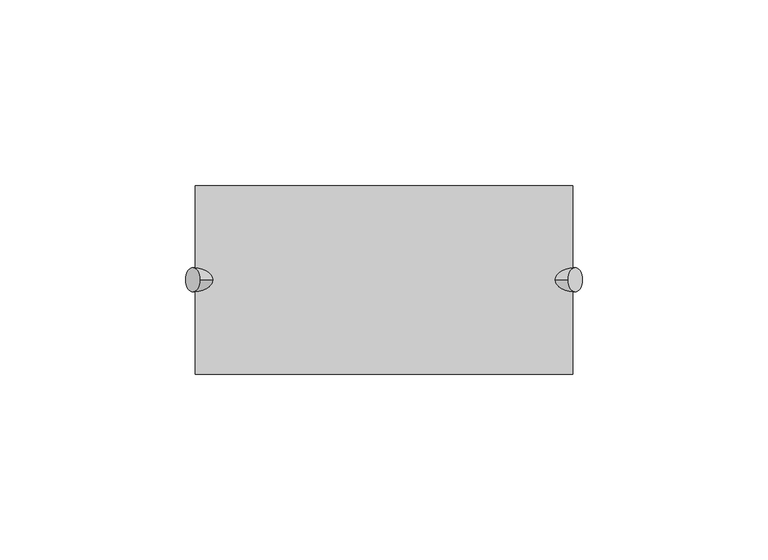
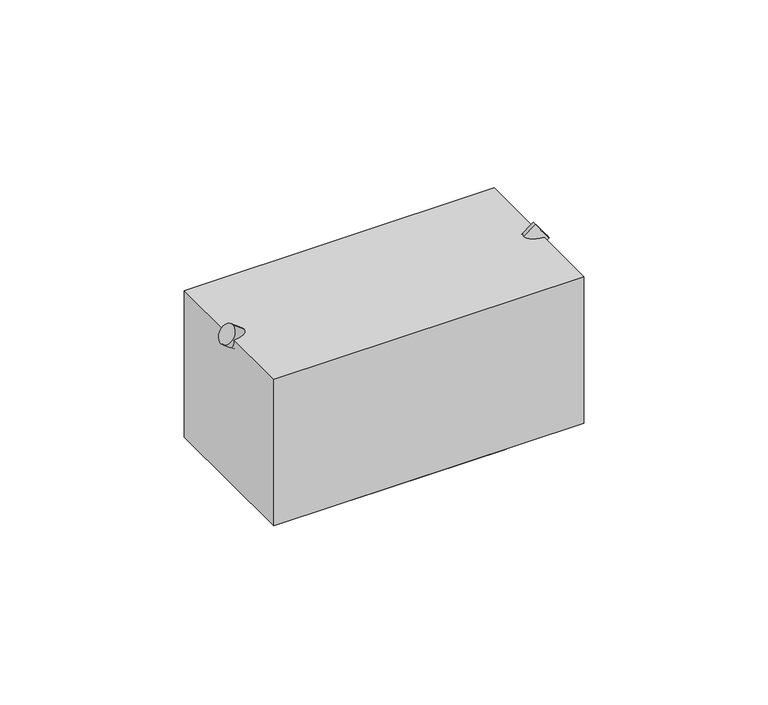
"""IFC4 building model written with IfcOpenShell, lengths in millimetres: proxy geometry, A5145 - Hook, Garment, Double : A5145 - Hook, Garment, Double."""

import ifcopenshell
import ifcopenshell.guid

model = None  # the IFC model being written
_history = None  # IfcOwnerHistory: only IFC2X3 demands one
_inside = {}  # id of a spatial element -> (the spatial element, [elements in it])
_under = {}  # id of a project, library or spatial element -> (it, [spatial elements below it])
_declared = {}  # id of a project -> (the project, [libraries it declares])
_typed = {}  # id of a type object -> (the type object, [elements of that type])
_made_of = {}  # id of a material, layer set ... -> (it, [elements and type objects made of it])


def new_model(schema):
    """Start an empty IFC model of exactly this schema.

    Asked for "IFC4X3", IfcOpenShell would pick the latest addendum, in which some entities
    have other attributes; the version numbers below select the first issue.
    IFC2X3 requires an IfcOwnerHistory on every rooted entity: one is made here for all.
    """
    global model, _history
    if schema == "IFC4X3":
        model = ifcopenshell.file(schema_version=(4, 3, 0, 0))
    else:
        model = ifcopenshell.file(schema=schema)
    _inside.clear()
    _under.clear()
    _declared.clear()
    _typed.clear()
    _made_of.clear()
    _history = None
    if model.schema == "IFC2X3":
        org = make("IfcOrganization", Name="unknown")
        user = make(
            "IfcPersonAndOrganization",
            ThePerson=make("IfcPerson", FamilyName="unknown"),
            TheOrganization=org,
        )
        app = make(
            "IfcApplication",
            ApplicationDeveloper=org,
            Version="unknown",
            ApplicationFullName="unknown",
            ApplicationIdentifier="unknown",
        )
        _history = make(
            "IfcOwnerHistory",
            OwningUser=user,
            OwningApplication=app,
            ChangeAction="ADDED",
            CreationDate=0,
        )
    return model


def make(cls, **values):
    """One entity of the class cls with the attributes given. An attribute that is None is left unset."""
    return model.create_entity(
        cls, **{name: value for name, value in values.items() if value is not None}
    )


def rooted(cls, **values):
    """An entity with a GlobalId (a new one), such as an element, a storey or a relation."""
    return make(cls, GlobalId=ifcopenshell.guid.new(), OwnerHistory=_history, **values)


def si_unit(unit_type, name, prefix=None):
    """IfcSIUnit, for example si_unit("LENGTHUNIT", "METRE", prefix="MILLI")."""
    return make("IfcSIUnit", UnitType=unit_type, Prefix=prefix, Name=name)


def assignment(units):
    """IfcUnitAssignment: the units of a project."""
    return None if units is None else make("IfcUnitAssignment", Units=units)


def point(xyz):
    """IfcCartesianPoint."""
    return None if xyz is None else make("IfcCartesianPoint", Coordinates=xyz)


def direction(xyz):
    """IfcDirection."""
    return None if xyz is None else make("IfcDirection", DirectionRatios=xyz)


def frame(location, z_axis=None, x_axis=None):
    """IfcAxis2Placement3D, a coordinate frame: its origin and axes. An axis left out is left unset."""
    return make(
        "IfcAxis2Placement3D",
        Location=point(location),
        Axis=direction(z_axis),
        RefDirection=direction(x_axis),
    )


def origin():
    """The frame at (0, 0, 0) with its axes left unset."""
    return frame((0.0, 0.0, 0.0))


def origin_with_axes():
    """The frame at (0, 0, 0) with the z axis (0, 0, 1) and the x axis (1, 0, 0) written out."""
    return frame((0.0, 0.0, 0.0), z_axis=(0.0, 0.0, 1.0), x_axis=(1.0, 0.0, 0.0))


def place(relative_to, where):
    """IfcLocalPlacement: puts the frame where relative to a parent placement (None: the world)."""
    return make(
        "IfcLocalPlacement", PlacementRelTo=relative_to, RelativePlacement=where
    )


def context(
    kind, dimensions, precision=None, world=None, true_north=None, identifier=None
):
    """IfcGeometricRepresentationContext, for example the 3D "Model" context."""
    return make(
        "IfcGeometricRepresentationContext",
        ContextIdentifier=identifier,
        ContextType=kind,
        CoordinateSpaceDimension=dimensions,
        Precision=precision,
        WorldCoordinateSystem=world,
        TrueNorth=true_north,
    )


def project(units=None, contexts=None):
    """IfcProject with its units and contexts."""
    return rooted(
        "IfcProject",
        Name="project",
        RepresentationContexts=contexts,
        UnitsInContext=assignment(units),
    )


def spatial(cls, under=None, at=None, **own):
    """A site, building, storey or space (cls), placed at a placement, below another one or the project."""
    s = rooted(cls, ObjectPlacement=at, **own)
    if under is not None:
        _under.setdefault(under.id(), (under, []))[1].append(s)
    return s


def polyline(points):
    """IfcPolyline through the points."""
    return make("IfcPolyline", Points=[point(p) for p in points])


def circle_curve(where, radius):
    """IfcCircle in the frame where."""
    return make("IfcCircle", Position=where, Radius=radius)


def ellipse_curve(where, semi_axis1, semi_axis2):
    """IfcEllipse in the frame where."""
    return make(
        "IfcEllipse", Position=where, SemiAxis1=semi_axis1, SemiAxis2=semi_axis2
    )


def outline(outer, holes=None, kind="AREA"):
    """IfcArbitraryClosedProfileDef: a profile drawn as a closed curve; with holes, ...WithVoids."""
    if holes is None:
        return make("IfcArbitraryClosedProfileDef", ProfileType=kind, OuterCurve=outer)
    return make(
        "IfcArbitraryProfileDefWithVoids",
        ProfileType=kind,
        OuterCurve=outer,
        InnerCurves=holes,
    )


def extrude(swept, where, along, depth):
    """IfcExtrudedAreaSolid: the profile swept, set in the frame where, extruded along a direction by depth."""
    return make(
        "IfcExtrudedAreaSolid",
        SweptArea=swept,
        Position=where,
        ExtrudedDirection=direction(along),
        Depth=depth,
    )


def shape(context_of_items, identifier, shape_type, items):
    """IfcShapeRepresentation: the items that make up one representation, for example the "Body"."""
    return make(
        "IfcShapeRepresentation",
        ContextOfItems=context_of_items,
        RepresentationIdentifier=identifier,
        RepresentationType=shape_type,
        Items=items,
    )


def source(mapping_origin, context_of_items, identifier, shape_type, items):
    """IfcRepresentationMap: a shape defined once, which mapped items show again and again."""
    return make(
        "IfcRepresentationMap",
        MappingOrigin=mapping_origin,
        MappedRepresentation=shape(context_of_items, identifier, shape_type, items),
    )


def transform(
    local_origin,
    x_axis=None,
    y_axis=None,
    z_axis=None,
    scale=None,
    scale2=None,
    scale3=None,
    uniform=True,
):
    """IfcCartesianTransformationOperator3D, or its non-uniform kind. x_axis, y_axis, z_axis: its Axis1, 2, 3."""
    if uniform:
        return make(
            "IfcCartesianTransformationOperator3D",
            Axis1=direction(x_axis),
            Axis2=direction(y_axis),
            LocalOrigin=point(local_origin),
            Scale=scale,
            Axis3=direction(z_axis),
        )
    return make(
        "IfcCartesianTransformationOperator3DnonUniform",
        Axis1=direction(x_axis),
        Axis2=direction(y_axis),
        LocalOrigin=point(local_origin),
        Scale=scale,
        Axis3=direction(z_axis),
        Scale2=scale2,
        Scale3=scale3,
    )


def mapped(mapping_source, mapping_target):
    """IfcMappedItem: shows the shape of a source again, moved by a transform."""
    return make(
        "IfcMappedItem", MappingSource=mapping_source, MappingTarget=mapping_target
    )


def made_of(thing, what):
    """Note that an element or type object is made of a material, layer set ...; save() writes the relation."""
    if what is not None:
        _made_of.setdefault(what.id(), (what, []))[1].append(thing)
    return thing


def element(
    cls,
    number,
    at=None,
    inside=None,
    cuts=None,
    type_object=None,
    material=None,
    context=None,
    identifier="Body",
    shape_type=None,
    held_by="IfcProductDefinitionShape",
    body=None,
    shapes=None,
    **own,
):
    """One element of the class cls, such as IfcWall. Its Tag is "e" and its number.

    at: its placement. inside: the storey or other place that contains it. cuts: it is an
    opening in that element (IfcRelVoidsElement). A single representation is given by context,
    identifier, shape_type and body (its items); several are given by shapes. held_by: the class
    of the entity that holds the representations. save() writes the other relations.
    """
    e = rooted(cls, Tag="e%d" % number, ObjectPlacement=at, **own)
    if body is not None:
        shapes = [shape(context, identifier, shape_type, body)]
    if shapes is not None:
        e.Representation = make(held_by, Representations=shapes)
    if inside is not None:
        _inside.setdefault(inside.id(), (inside, []))[1].append(e)
    if cuts is not None:
        rooted(
            "IfcRelVoidsElement", RelatingBuildingElement=cuts, RelatedOpeningElement=e
        )
    if type_object is not None:
        _typed.setdefault(type_object.id(), (type_object, []))[1].append(e)
    return made_of(e, material)


def aggregate(whole, parts):
    """IfcRelAggregates: a whole, such as a stair, and the parts it consists of."""
    return rooted("IfcRelAggregates", RelatingObject=whole, RelatedObjects=parts)


def save(model, path):
    """Write the relations noted so far, then the file.

    IfcRelAggregates (storeys below a building ...), IfcRelContainedInSpatialStructure (elements
    in a storey), IfcRelDefinesByType, IfcRelAssociatesMaterial and IfcRelDeclares: one each for
    every whole, place, type object, material and project.
    """
    for whole, parts in _under.values():
        aggregate(whole, parts)
    for where, things in _inside.values():
        rooted(
            "IfcRelContainedInSpatialStructure",
            RelatedElements=things,
            RelatingStructure=where,
        )
    for kind, things in _typed.values():
        rooted("IfcRelDefinesByType", RelatedObjects=things, RelatingType=kind)
    for what, things in _made_of.values():
        rooted("IfcRelAssociatesMaterial", RelatedObjects=things, RelatingMaterial=what)
    for by, libraries in _declared.values():
        rooted("IfcRelDeclares", RelatingContext=by, RelatedDefinitions=libraries)
    model.write(path)


def plane_surface(at):
    """IfcPlane: the flat surface through the origin of the frame at, square to its z axis."""
    return make("IfcPlane", Position=at)


def cylinder_surface(at, radius):
    """IfcCylindricalSurface: all points at the distance radius from the z axis of the frame at."""
    return make("IfcCylindricalSurface", Position=at, Radius=radius)


def advanced_brep(points, edges, surfaces, faces):
    """IfcAdvancedBrep: a solid bounded by faces that lie on surfaces and meet in shared edges.

    An edge is (start, end): straight between two places in points (the first is 0);
    or (start, end, curve); or (start, end, curve, False) where it runs against its curve.
    A face is (place in surfaces, loops), or (place, loops, False) where it looks against
    its surface's normal. A loop lists edges by number (the first is 1), with a minus sign
    where the edge is run from its end to its start. The first loop is the outer one.
    """
    corners = [point(p) for p in points]
    vertices = [make("IfcVertexPoint", VertexGeometry=c) for c in corners]
    made = []
    for start, end, *more in edges:
        made.append(
            make(
                "IfcEdgeCurve",
                EdgeStart=vertices[start],
                EdgeEnd=vertices[end],
                EdgeGeometry=more[0] if more else make("IfcPolyline", Points=[corners[start], corners[end]]),
                SameSense=more[1] if len(more) > 1 else True,
            )
        )
    hull = []
    for where, loops, *sense in faces:
        bounds = []
        for j, loop in enumerate(loops):
            ring = [make("IfcOrientedEdge", EdgeElement=made[abs(k) - 1], Orientation=k > 0) for k in loop]
            bounds.append(
                make(
                    "IfcFaceOuterBound" if j == 0 else "IfcFaceBound",
                    Bound=make("IfcEdgeLoop", EdgeList=ring),
                    Orientation=True,
                )
            )
        hull.append(make("IfcAdvancedFace", Bounds=bounds, FaceSurface=surfaces[where], SameSense=sense[0] if sense else True))
    return make("IfcAdvancedBrep", Outer=make("IfcClosedShell", CfsFaces=hull))


def specialty_equipment_dbff7740(model_context):
    return source(origin(), model_context, "Body", "SolidModel", [
        extrude(outline(polyline([(50.8, -25.4), (-50.8, -25.4), (-50.8, 25.4), (50.8, 25.4), (50.8, -25.4)])), origin_with_axes(), (0.0, 0.0, 1.0), 50.8),
        advanced_brep(
        [(-53.475253, 0.0, 48.7696452), (-49.5999303, 0.0, 53.9367422), (0.0, 0.0, 16.7367945), (0.0, 3.2294356, 12.7), (-5.3823927, 0.0, 12.7), (0.0, -3.2294356, 12.7), (53.475253, 0.0, 48.7696452), (49.5999303, 0.0, 53.9367422), (5.3823927, 0.0, 12.7), (-25.4, 25.4, 12.7), (-25.4, -25.4, 12.7), (25.4, -25.4, 12.7), (25.4, 25.4, 12.7), (-25.4, 25.4, 0.0), (25.4, 25.4, 0.0), (25.4, -25.4, 0.0), (-25.4, -25.4, 0.0)],
        [
            (0, 1, circle_curve(frame((-51.5375917, 0.0, 51.3531937), z_axis=(-0.7999999999999928, 0.0, 0.6000000000000097), x_axis=(0.6000000000000097, 0.0, 0.7999999999999928)), 3.2294356)),
            (1, 0, circle_curve(frame((-51.5375917, 0.0, 51.3531937), z_axis=(-0.7999999999999928, 0.0, 0.6000000000000097), x_axis=(0.6000000000000097, 0.0, 0.7999999999999928)), 3.2294356)),
            (1, 2),
            (2, 3, ellipse_curve(frame((0.0, 0.0, 12.7), z_axis=(-0.9999999999999999, 0.0, 0.0), x_axis=(0.0, 0.0, 1.0)), 4.0367945, 3.2294356)),
            (3, 4, ellipse_curve(frame((0.0, 0.0, 12.7), z_axis=(0.0, 0.0, 1.0), x_axis=(-0.9999999999999999, 0.0, 0.0)), 5.3823927, 3.2294356)),
            (4, 0),
            (4, 5, ellipse_curve(frame((0.0, 0.0, 12.7), z_axis=(0.0, 0.0, 1.0), x_axis=(-0.9999999999999999, 0.0, 0.0)), 5.3823927, 3.2294356)),
            (5, 2, ellipse_curve(frame((0.0, 0.0, 12.7), z_axis=(-0.9999999999999999, 0.0, 0.0), x_axis=(0.0, 0.0, 1.0)), 4.0367945, 3.2294356)),
            (6, 7, circle_curve(frame((51.5375917, 0.0, 51.3531937), z_axis=(0.7999999999999928, 0.0, 0.6000000000000097), x_axis=(-0.6000000000000097, 0.0, 0.7999999999999928)), 3.2294356)),
            (7, 6, circle_curve(frame((51.5375917, 0.0, 51.3531937), z_axis=(0.7999999999999928, 0.0, 0.6000000000000097), x_axis=(-0.6000000000000097, 0.0, 0.7999999999999928)), 3.2294356)),
            (6, 8),
            (8, 3, ellipse_curve(frame((0.0, 0.0, 12.7), z_axis=(0.0, 0.0, 1.0), x_axis=(0.9999999999999999, 0.0, 0.0)), 5.3823927, 3.2294356)),
            (2, 7),
            (5, 8, ellipse_curve(frame((0.0, 0.0, 12.7), z_axis=(0.0, 0.0, 1.0), x_axis=(0.9999999999999999, 0.0, 0.0)), 5.3823927, 3.2294356)),
            (9, 10),
            (10, 11),
            (11, 12),
            (12, 9),
            (13, 14),
            (14, 15),
            (15, 16),
            (16, 13),
            (9, 13),
            (16, 10),
            (15, 11),
            (14, 12),
        ],
        [
            plane_surface(frame((-49.5999303, 0.0, 53.9367422), z_axis=(-0.7999999999999927, 0.0, 0.6000000000000097), x_axis=(0.0, -1.0, 0.0))),
            cylinder_surface(frame((0.0, 0.0, 12.7), z_axis=(-0.7999999999999928, 0.0, 0.6000000000000097), x_axis=(0.6000000000000097, 0.0, 0.7999999999999928)), 3.2294356),
            plane_surface(frame((49.5999303, 0.0, 53.9367422), z_axis=(0.7999999999999927, 0.0, 0.6000000000000097), x_axis=(0.0, 1.0, 0.0))),
            cylinder_surface(frame((0.0, 0.0, 12.7), z_axis=(0.7999999999999928, 0.0, 0.6000000000000097), x_axis=(-0.6000000000000097, 0.0, 0.7999999999999928)), 3.2294356),
            plane_surface(frame((25.4, 25.4, 12.7), z_axis=(0.0, 0.0, 1.0), x_axis=(1.0, 0.0, 0.0))),
            plane_surface(frame((25.4, 25.4, 0.0), z_axis=(0.0, 0.0, -1.0), x_axis=(-1.0, 0.0, 0.0))),
            plane_surface(frame((-25.4, -25.4, 12.7), z_axis=(-1.0, 0.0, 0.0), x_axis=(0.0, 0.0, -1.0))),
            plane_surface(frame((25.4, -25.4, 12.7), z_axis=(0.0, -1.0, 0.0), x_axis=(0.0, 0.0, -1.0))),
            plane_surface(frame((25.4, 25.4, 12.7), z_axis=(1.0, 0.0, 0.0), x_axis=(0.0, 0.0, -1.0))),
            plane_surface(frame((-25.4, 25.4, 12.7), z_axis=(0.0, 1.0, 0.0), x_axis=(0.0, 0.0, -1.0))),
        ],
        [
            (0, [[1, 2]]),
            (1, [[3, 4, 5, 6, -2]]),
            (1, [[-6, 7, 8, -3, -1]]),
            (2, [[9, 10]]),
            (3, [[11, 12, -4, 13, -9]]),
            (3, [[-13, -8, 14, -11, -10]]),
            (4, [[15, 16, 17, 18], [-12, -14, -7, -5]]),
            (5, [[19, 20, 21, 22]]),
            (6, [[23, -22, 24, -15]]),
            (7, [[-24, -21, 25, -16]]),
            (8, [[-25, -20, 26, -17]]),
            (9, [[-26, -19, -23, -18]]),
        ],
    ),
    ])


if __name__ == "__main__":
    model = new_model("IFC4")
    model_context = context("Model", 3, world=origin())
    ifc_project = project(units=[si_unit("LENGTHUNIT", "METRE", prefix="MILLI")], contexts=[model_context])
    site = spatial("IfcSite", under=ifc_project)
    building = spatial("IfcBuilding", under=site)
    placement = place(None, origin())
    specialty_equipment_shape = specialty_equipment_dbff7740(model_context)
    element("IfcBuildingElementProxy", 1, Name="A5145 - Hook, Garment, Double : A5145 - Hook, Garment, Double", ObjectType="A5145 - Hook, Garment, Double : A5145 - Hook, Garment, Double", at=placement, inside=building, context=model_context, shape_type="MappedRepresentation", body=[
        mapped(specialty_equipment_shape, transform((0.0, 0.0, 0.0), x_axis=(1.0, 0.0, 0.0), y_axis=(0.0, 1.0, 0.0), z_axis=(0.0, 0.0, 1.0))),
    ])
    save(model, "model.ifc")

# Revit data of these elements
# Type "A5145 - Hook, Garment, Double : A5145 - Hook, Garment, Double"
#   Watts2 = "0"
#   Watts1 = "0"
#   Unit_Issue = "EA"
#   UTIL_6_Misc = "-"
#   UTIL_5_NonMedGas = "-"
#   UTIL_4_MiscGas = "-"
#   UTIL_3_MedGas = "-"
#   UTIL_2_Elec = "-"
#   UTIL_1_WaterDrain = "-"
#   Nomenclature = "Hook, Garment, Double, SS, Surface Mounted"
#   NSN = "5340007541678"
#   Location [instance default] = ""
#   JSN = "A5145"
#   Fund_Source_VA = "-"
#   Fund_Source_Navy = "-"
#   Fund_Source_Army = "-"
#   Fund_Source_AF = "-"
#   ELEC_Volts2 = "0"
#   ELEC_Volts1 = "0"
#   ELEC_Phase2 = "0"
#   ELEC_Phase1 = "0"
#   ELEC_HertzSwitch = "0"
#   ELEC_HertzDependent = "0"
#   ELEC_Hertz = "0"
#   ELEC_Amps2 = "0"
#   ELEC_Amps1 = "0"
#   DetailDescription = "A surface mounted, satin finish stainless steel, double garment hook. Equipped with a concealed mounting bracket that is secured to a concealed wall plate. For general purpose use throughout the facility to hang various items of apparel."
#   CAT_VA = "A"
#   CAT_Navy = "A"
#   CAT_IHS = "-"
#   CAT_Army = "A"
#   CAT_AF = "A"
#   BTUperhour = "0"
#   Weight_IP = 0
#   Default Elevation = 4' - 6"
#   DIM_Width_IP = 0' - 4"
#   DIM_Height_IP = 0' - 2"
#   DIM_Depth_IP = 0' - 2"
#   Assembly Code = ""
# Element 1 (IfcBuildingElementProxy, "A5145 - Hook, Garment, Double : A5145 - Hook, Garment, Double")
#   Location = "BRAR2"
#   Materials on its faces: "EquipSpace"
# Materials
#   "EquipSpace": class "Unassigned", colour RGB 221 217 195, transparency 0.5
